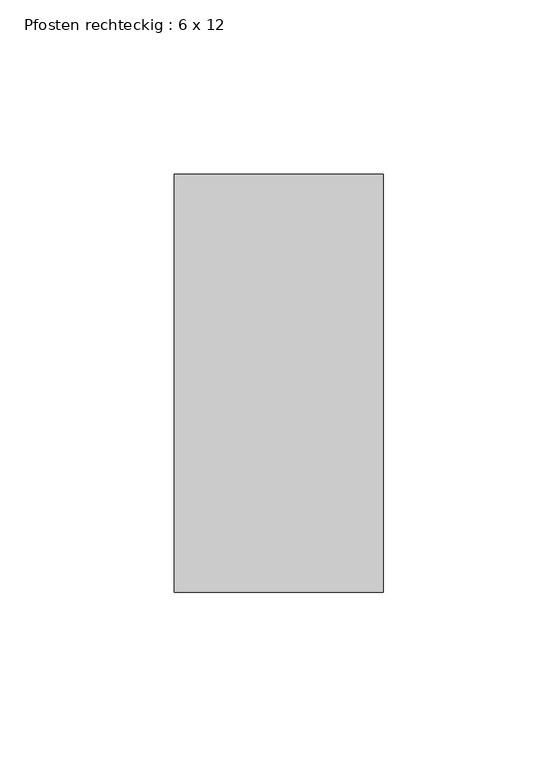
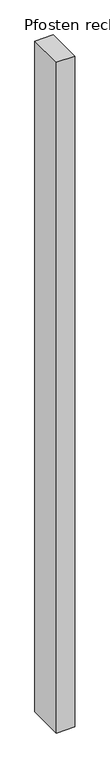
"""IFC4 building model written with IfcOpenShell, lengths in millimetres: member geometry, Pfosten rechteckig : 6 x 12."""

from ifc_helpers import new_model, si_unit, frame, origin, place, context, project, spatial, polyline, outline, extrude, source, transform, mapped, element, save


def pfosten_rechteckig_6_x_12_6681f09f(model_context):
    return source(origin(), model_context, "Body", "SweptSolid", [
        extrude(outline(polyline([(30.0, 60.0), (30.0, -60.0), (-30.0, -60.0), (-30.0, 60.0), (30.0, 60.0)])), frame((0.0, 0.0, -2290.8558388), z_axis=(0.0, 0.0, 1.0), x_axis=(1.0, 0.0, 0.0)), (0.0, 0.0, 1.0), 2290.8558388),
    ])


if __name__ == "__main__":
    model = new_model("IFC4")
    model_context = context("Model", 3, world=origin())
    ifc_project = project(units=[si_unit("LENGTHUNIT", "METRE", prefix="MILLI")], contexts=[model_context])
    site = spatial("IfcSite", under=ifc_project)
    building = spatial("IfcBuilding", under=site)
    placement = place(None, origin())
    pfosten_rechteckig_6_x_12_shape = pfosten_rechteckig_6_x_12_6681f09f(model_context)
    element("IfcMember", 1, ObjectType="Pfosten rechteckig : 6 x 12", at=placement, inside=building, context=model_context, shape_type="MappedRepresentation", body=[
        mapped(pfosten_rechteckig_6_x_12_shape, transform((0.0, 0.0, 0.0), x_axis=(1.0, 0.0, 0.0), y_axis=(0.0, 1.0, 0.0), z_axis=(0.0, 0.0, 1.0))),
    ])
    save(model, "model.ifc")

# Revit data of these elements
# Type "Pfosten rechteckig : 6 x 12"
#   built-in parameter 1007304 = 0.393701 (stored number, unit not read)
#   built-in parameter 1007301 = 0.0984252 (stored number, unit not read)
#   built-in parameter 1007300 = 0.0984252 (stored number, unit not read)
# Element 1 (IfcMember, "Pfosten rechteckig : 6 x 12")
#   Materials on its faces: "Metall - verzinkt"
# Materials
#   "Metall - verzinkt": class "Allgemeines", colour RGB 200 200 200, transparency 0, Cost = 0
